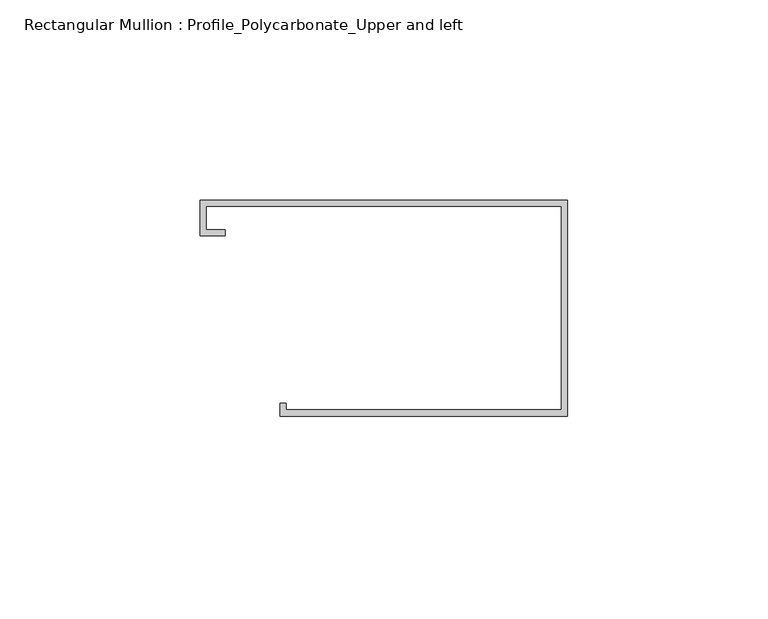
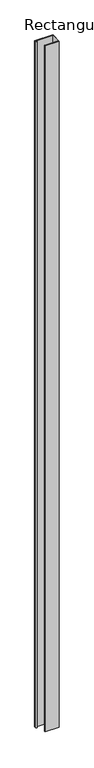
"""IFC4 building model written with IfcOpenShell, lengths in millimetres: member geometry, Rectangular Mullion : Profile_Polycarbonate_Upper and left."""

from ifc_helpers import new_model, si_unit, frame, origin, place, context, project, spatial, polyline, outline, extrude, source, transform, mapped, element, save


def rectangular_mullion_profile_polycarbonate_upper_and_left_46bbe178(model_context):
    return source(origin(), model_context, "Body", "SweptSolid", [
        extrude(outline(polyline([(0.0, 28.984575), (0.0, -25.015825), (-71.9836, -25.015825), (-71.9836, -21.840825), (-70.3961, -21.840825), (-70.3961, -23.428325), (-1.5875, -23.428325), (-1.5875, 27.397075), (-90.4113, 27.397075), (-90.4113, 21.580475), (-85.6488, 21.580475), (-85.6488, 19.992975), (-91.9988, 19.992975), (-91.9988, 28.984575), (0.0, 28.984575)])), frame((0.0, 0.0, -3657.6), z_axis=(0.0, 0.0, 1.0), x_axis=(1.0, 0.0, 0.0)), (0.0, 0.0, 1.0), 3657.6),
    ])


if __name__ == "__main__":
    model = new_model("IFC4")
    model_context = context("Model", 3, world=origin())
    ifc_project = project(units=[si_unit("LENGTHUNIT", "METRE", prefix="MILLI")], contexts=[model_context])
    site = spatial("IfcSite", under=ifc_project)
    building = spatial("IfcBuilding", under=site)
    placement = place(None, origin())
    rectangular_mullion_profile_polycarbonate_upper_and_left_shape = rectangular_mullion_profile_polycarbonate_upper_and_left_46bbe178(model_context)
    element("IfcMember", 1, ObjectType="Rectangular Mullion : Profile_Polycarbonate_Upper and left", at=placement, inside=building, context=model_context, shape_type="MappedRepresentation", body=[
        mapped(rectangular_mullion_profile_polycarbonate_upper_and_left_shape, transform((0.0, 0.0, 0.0), x_axis=(1.0, 0.0, 0.0), y_axis=(0.0, 1.0, 0.0), z_axis=(0.0, 0.0, 1.0))),
    ])
    save(model, "model.ifc")

# Revit data of these elements
# Type "Rectangular Mullion : Profile_Polycarbonate_Upper and left"
#   built-in parameter 1007322 = 0.177167 (stored number, unit not read)
#   built-in parameter 1007321 = 0.00520833 (stored number, unit not read)
#   built-in parameter 1007320 = 0 (stored number, unit not read)
